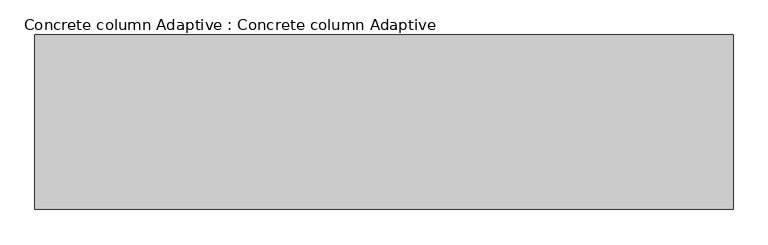
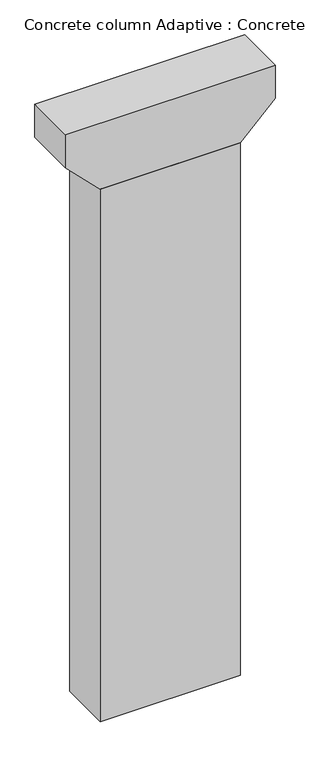
"""IFC4 building model written with IfcOpenShell, lengths in millimetres: proxy geometry, Concrete column Adaptive : Concrete column Adaptive."""

from ifc_helpers import new_model, si_unit, frame, origin, origin_with_axes, place, context, project, spatial, polyline, outline, extrude, source, transform, mapped, element, save


def concrete_column_adaptive_concrete_column_adaptive_8623096c(model_context):
    return source(origin(), model_context, "Body", "SweptSolid", [
        extrude(outline(polyline([(36183.0, 6000.0), (36183.0, -6000.0), (34183.0, -6000.0), (32183.0, -4000.0), (32183.0, 4000.0), (34183.0, 6000.0), (36183.0, 6000.0)])), frame((0.0, -1500.0, 0.0), z_axis=(0.0, 1.0, 0.0), x_axis=(0.0, 0.0, 1.0)), (0.0, 0.0, 1.0), 3000.0),
        extrude(outline(polyline([(-4000.0, -1500.0), (-4000.0, 1500.0), (4000.0, 1500.0), (4000.0, -1500.0), (-4000.0, -1500.0)])), origin_with_axes(), (0.0, 0.0, 1.0), 32183.0),
    ])


if __name__ == "__main__":
    model = new_model("IFC4")
    model_context = context("Model", 3, world=origin())
    ifc_project = project(units=[si_unit("LENGTHUNIT", "METRE", prefix="MILLI")], contexts=[model_context])
    site = spatial("IfcSite", under=ifc_project)
    building = spatial("IfcBuilding", under=site)
    placement = place(None, origin())
    concrete_column_adaptive_concrete_column_adaptive_shape = concrete_column_adaptive_concrete_column_adaptive_8623096c(model_context)
    element("IfcBuildingElementProxy", 1, Name="Concrete column Adaptive : Concrete column Adaptive", ObjectType="Concrete column Adaptive : Concrete column Adaptive", at=placement, inside=building, context=model_context, shape_type="MappedRepresentation", body=[
        mapped(concrete_column_adaptive_concrete_column_adaptive_shape, transform((0.0, 0.0, 0.0), x_axis=(1.0, 0.0, 0.0), y_axis=(0.0, 1.0, 0.0), z_axis=(0.0, 0.0, 1.0))),
    ])
    save(model, "model.ifc")

# Revit data of these elements
# Type "Concrete column Adaptive : Concrete column Adaptive"
#   Height [instance default] = 30000 mm
#   Default Elevation = 0
# Element 1 (IfcBuildingElementProxy, "Concrete column Adaptive : Concrete column Adaptive")
#   Height = 32183 mm
